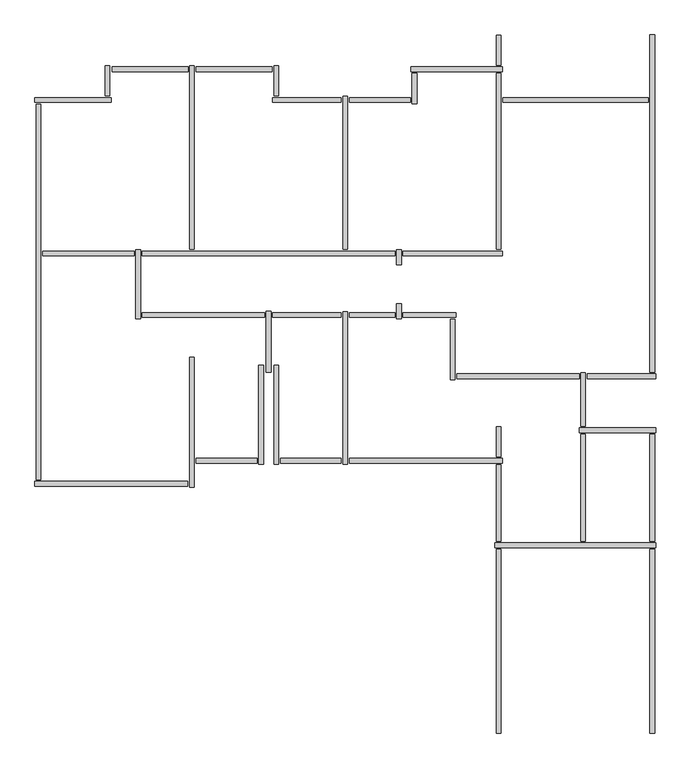
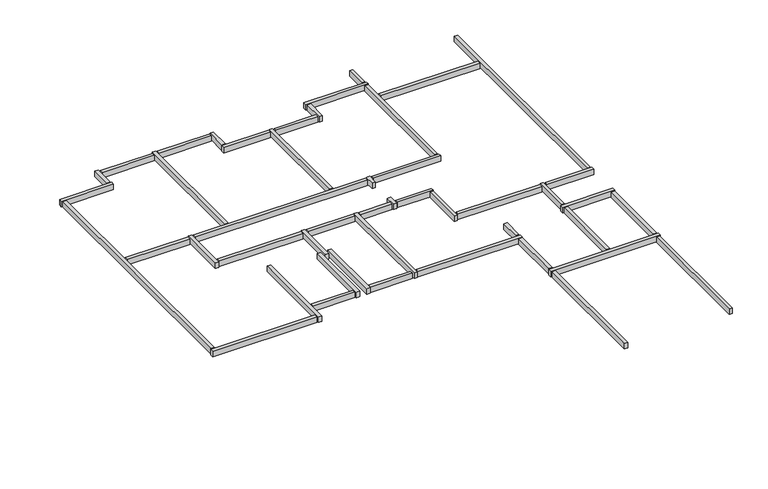
"""IFC4 building model written with IfcOpenShell, lengths in millimetres: beam geometry, Graute viga de respaldo23 : Graute viga de respaldo."""

from ifc_helpers import new_model, si_unit, frame, origin, place, context, project, spatial, polyline, outline, extrude, source, transform, mapped, element, save


def beam_4ae021a0(model_context):
    return source(origin(), model_context, "Body", "SweptSolid", [
        extrude(outline(polyline([(-70718.7587292, 62785.4278788), (-70624.7587292, 62785.4278788), (-70624.7587292, 59195.4278788), (-70718.7587292, 59195.4278788), (-70718.7587292, 62785.4278788)])), frame((0.0, 0.0, 17632.9999999), z_axis=(0.0, 0.0, 1.0), x_axis=(1.0, 0.0, 0.0)), (0.0, 0.0, 1.0), 167.0),
        extrude(outline(polyline([(-67718.7587292, 62785.4278788), (-67624.7587292, 62785.4278788), (-67624.7587292, 59195.4278788), (-67718.7587292, 59195.4278788), (-67718.7587292, 62785.4278788)])), frame((0.0, 0.0, 17632.9999999), z_axis=(0.0, 0.0, 1.0), x_axis=(1.0, 0.0, 0.0)), (0.0, 0.0, 1.0), 167.0),
        extrude(outline(polyline([(-75401.7587292, 64562.4278788), (-75401.7587292, 64468.4278788), (-76591.7587292, 64468.4278788), (-76591.7587292, 64562.4278788), (-75401.7587292, 64562.4278788)])), frame((0.0, 0.0, 17632.9999999), z_axis=(0.0, 0.0, 1.0), x_axis=(1.0, 0.0, 0.0)), (0.0, 0.0, 1.0), 167.0),
        extrude(outline(polyline([(-73751.7587292, 64562.4278788), (-73751.7587292, 64468.4278788), (-74941.7587292, 64468.4278788), (-74941.7587292, 64562.4278788), (-73751.7587292, 64562.4278788)])), frame((0.0, 0.0, 17632.9999999), z_axis=(0.0, 0.0, 1.0), x_axis=(1.0, 0.0, 0.0)), (0.0, 0.0, 1.0), 167.0),
        extrude(outline(polyline([(-77801.7587292, 68612.4278788), (-77801.7587292, 68518.4278788), (-79591.7587292, 68518.4278788), (-79591.7587292, 68612.4278788), (-77801.7587292, 68612.4278788)])), frame((0.0, 0.0, 17632.9999999), z_axis=(0.0, 0.0, 1.0), x_axis=(1.0, 0.0, 0.0)), (0.0, 0.0, 1.0), 167.0),
        extrude(outline(polyline([(-72401.7587292, 71612.4278788), (-72401.7587292, 71518.4278788), (-73591.7587292, 71518.4278788), (-73591.7587292, 71612.4278788), (-72401.7587292, 71612.4278788)])), frame((0.0, 0.0, 17632.9999999), z_axis=(0.0, 0.0, 1.0), x_axis=(1.0, 0.0, 0.0)), (0.0, 0.0, 1.0), 167.0),
        extrude(outline(polyline([(-72274.7587292, 71495.4278788), (-72368.7587292, 71495.4278788), (-72368.7587292, 72085.4278788), (-72274.7587292, 72085.4278788), (-72274.7587292, 71495.4278788)])), frame((0.0, 0.0, 17632.9999999), z_axis=(0.0, 0.0, 1.0), x_axis=(1.0, 0.0, 0.0)), (0.0, 0.0, 1.0), 167.0),
        extrude(outline(polyline([(-70601.7587292, 72212.4278788), (-70601.7587292, 72118.4278788), (-72391.7587292, 72118.4278788), (-72391.7587292, 72212.4278788), (-70601.7587292, 72212.4278788)])), frame((0.0, 0.0, 17632.9999999), z_axis=(0.0, 0.0, 1.0), x_axis=(1.0, 0.0, 0.0)), (0.0, 0.0, 1.0), 167.0),
        extrude(outline(polyline([(-72668.7587292, 68635.4278788), (-72574.7587292, 68635.4278788), (-72574.7587292, 68345.4278788), (-72668.7587292, 68345.4278788), (-72668.7587292, 68635.4278788)])), frame((0.0, 0.0, 17632.9999999), z_axis=(0.0, 0.0, 1.0), x_axis=(1.0, 0.0, 0.0)), (0.0, 0.0, 1.0), 167.0),
        extrude(outline(polyline([(-75251.7587292, 67412.4278788), (-75251.7587292, 67318.4278788), (-77641.7587292, 67318.4278788), (-77641.7587292, 67412.4278788), (-75251.7587292, 67412.4278788)])), frame((0.0, 0.0, 17632.9999999), z_axis=(0.0, 0.0, 1.0), x_axis=(1.0, 0.0, 0.0)), (0.0, 0.0, 1.0), 167.0),
        extrude(outline(polyline([(-73751.7587292, 67412.4278788), (-73751.7587292, 67318.4278788), (-75091.7587292, 67318.4278788), (-75091.7587292, 67412.4278788), (-73751.7587292, 67412.4278788)])), frame((0.0, 0.0, 17632.9999999), z_axis=(0.0, 0.0, 1.0), x_axis=(1.0, 0.0, 0.0)), (0.0, 0.0, 1.0), 167.0),
        extrude(outline(polyline([(-72701.7587292, 67412.4278788), (-72701.7587292, 67318.4278788), (-73591.7587292, 67318.4278788), (-73591.7587292, 67412.4278788), (-72701.7587292, 67412.4278788)])), frame((0.0, 0.0, 17632.9999999), z_axis=(0.0, 0.0, 1.0), x_axis=(1.0, 0.0, 0.0)), (0.0, 0.0, 1.0), 167.0),
        extrude(outline(polyline([(-72668.7587292, 67585.4278788), (-72574.7587292, 67585.4278788), (-72574.7587292, 67295.4278788), (-72668.7587292, 67295.4278788), (-72668.7587292, 67585.4278788)])), frame((0.0, 0.0, 17632.9999999), z_axis=(0.0, 0.0, 1.0), x_axis=(1.0, 0.0, 0.0)), (0.0, 0.0, 1.0), 167.0),
        extrude(outline(polyline([(-71511.7587292, 67412.4278788), (-71511.7587292, 67318.4278788), (-72541.7587292, 67318.4278788), (-72541.7587292, 67412.4278788), (-71511.7587292, 67412.4278788)])), frame((0.0, 0.0, 17632.9999999), z_axis=(0.0, 0.0, 1.0), x_axis=(1.0, 0.0, 0.0)), (0.0, 0.0, 1.0), 167.0),
        extrude(outline(polyline([(-71524.7587292, 66095.4278788), (-71618.7587292, 66095.4278788), (-71618.7587292, 67285.4278788), (-71524.7587292, 67285.4278788), (-71524.7587292, 66095.4278788)])), frame((0.0, 0.0, 17632.9999999), z_axis=(0.0, 0.0, 1.0), x_axis=(1.0, 0.0, 0.0)), (0.0, 0.0, 1.0), 167.0),
        extrude(outline(polyline([(-69091.7587292, 66212.4278788), (-69091.7587292, 66118.4278788), (-71491.7587292, 66118.4278788), (-71491.7587292, 66212.4278788), (-69091.7587292, 66212.4278788)])), frame((0.0, 0.0, 17632.9999999), z_axis=(0.0, 0.0, 1.0), x_axis=(1.0, 0.0, 0.0)), (0.0, 0.0, 1.0), 167.0),
        extrude(outline(polyline([(-73718.7587292, 67430.4278788), (-73624.7587292, 67430.4278788), (-73624.7587292, 64445.4278788), (-73718.7587292, 64445.4278788), (-73718.7587292, 67430.4278788)])), frame((0.0, 0.0, 17632.9999999), z_axis=(0.0, 0.0, 1.0), x_axis=(1.0, 0.0, 0.0)), (0.0, 0.0, 1.0), 167.0),
        extrude(outline(polyline([(-70601.7587292, 64562.4278788), (-70601.7587292, 64468.4278788), (-73591.7587292, 64468.4278788), (-73591.7587292, 64562.4278788), (-70601.7587292, 64562.4278788)])), frame((0.0, 0.0, 17632.9999999), z_axis=(0.0, 0.0, 1.0), x_axis=(1.0, 0.0, 0.0)), (0.0, 0.0, 1.0), 167.0),
        extrude(outline(polyline([(-70718.7587292, 65185.4278788), (-70624.7587292, 65185.4278788), (-70624.7587292, 64595.4278788), (-70718.7587292, 64595.4278788), (-70718.7587292, 65185.4278788)])), frame((0.0, 0.0, 17632.9999999), z_axis=(0.0, 0.0, 1.0), x_axis=(1.0, 0.0, 0.0)), (0.0, 0.0, 1.0), 167.0),
        extrude(outline(polyline([(-70624.7587292, 62945.4278788), (-70718.7587292, 62945.4278788), (-70718.7587292, 64435.4278788), (-70624.7587292, 64435.4278788), (-70624.7587292, 62945.4278788)])), frame((0.0, 0.0, 17632.9999999), z_axis=(0.0, 0.0, 1.0), x_axis=(1.0, 0.0, 0.0)), (0.0, 0.0, 1.0), 167.0),
        extrude(outline(polyline([(-67624.7587292, 62945.4278788), (-67718.7587292, 62945.4278788), (-67718.7587292, 65035.4278788), (-67624.7587292, 65035.4278788), (-67624.7587292, 62945.4278788)])), frame((0.0, 0.0, 17632.9999999), z_axis=(0.0, 0.0, 1.0), x_axis=(1.0, 0.0, 0.0)), (0.0, 0.0, 1.0), 167.0),
        extrude(outline(polyline([(-68974.7587292, 62945.4278788), (-69068.7587292, 62945.4278788), (-69068.7587292, 65035.4278788), (-68974.7587292, 65035.4278788), (-68974.7587292, 62945.4278788)])), frame((0.0, 0.0, 17632.9999999), z_axis=(0.0, 0.0, 1.0), x_axis=(1.0, 0.0, 0.0)), (0.0, 0.0, 1.0), 167.0),
        extrude(outline(polyline([(-69068.7587292, 66235.4278788), (-68974.7587292, 66235.4278788), (-68974.7587292, 65195.4278788), (-69068.7587292, 65195.4278788), (-69068.7587292, 66235.4278788)])), frame((0.0, 0.0, 17632.9999999), z_axis=(0.0, 0.0, 1.0), x_axis=(1.0, 0.0, 0.0)), (0.0, 0.0, 1.0), 167.0),
        extrude(outline(polyline([(-67751.7587292, 71612.4278788), (-67751.7587292, 71518.4278788), (-70591.7587292, 71518.4278788), (-70591.7587292, 71612.4278788), (-67751.7587292, 71612.4278788)])), frame((0.0, 0.0, 17632.9999999), z_axis=(0.0, 0.0, 1.0), x_axis=(1.0, 0.0, 0.0)), (0.0, 0.0, 1.0), 167.0),
        extrude(outline(polyline([(-70624.7587292, 68645.4278788), (-70718.7587292, 68645.4278788), (-70718.7587292, 72085.4278788), (-70624.7587292, 72085.4278788), (-70624.7587292, 68645.4278788)])), frame((0.0, 0.0, 17632.9999999), z_axis=(0.0, 0.0, 1.0), x_axis=(1.0, 0.0, 0.0)), (0.0, 0.0, 1.0), 167.0),
        extrude(outline(polyline([(-70601.7587292, 68612.4278788), (-70601.7587292, 68518.4278788), (-72541.7587292, 68518.4278788), (-72541.7587292, 68612.4278788), (-70601.7587292, 68612.4278788)])), frame((0.0, 0.0, 17632.9999999), z_axis=(0.0, 0.0, 1.0), x_axis=(1.0, 0.0, 0.0)), (0.0, 0.0, 1.0), 167.0),
        extrude(outline(polyline([(-72701.7587292, 68612.4278788), (-72701.7587292, 68518.4278788), (-77641.7587292, 68518.4278788), (-77641.7587292, 68612.4278788), (-72701.7587292, 68612.4278788)])), frame((0.0, 0.0, 17632.9999999), z_axis=(0.0, 0.0, 1.0), x_axis=(1.0, 0.0, 0.0)), (0.0, 0.0, 1.0), 167.0),
        extrude(outline(polyline([(-73718.7587292, 71635.4278788), (-73624.7587292, 71635.4278788), (-73624.7587292, 68645.4278788), (-73718.7587292, 68645.4278788), (-73718.7587292, 71635.4278788)])), frame((0.0, 0.0, 17632.9999999), z_axis=(0.0, 0.0, 1.0), x_axis=(1.0, 0.0, 0.0)), (0.0, 0.0, 1.0), 167.0),
        extrude(outline(polyline([(-75091.7587292, 71518.4278788), (-75091.7587292, 71612.4278788), (-73751.7587292, 71612.4278788), (-73751.7587292, 71518.4278788), (-75091.7587292, 71518.4278788)])), frame((0.0, 0.0, 17632.9999999), z_axis=(0.0, 0.0, 1.0), x_axis=(1.0, 0.0, 0.0)), (0.0, 0.0, 1.0), 167.0),
        extrude(outline(polyline([(-75068.7587292, 72235.4278788), (-74974.7587292, 72235.4278788), (-74974.7587292, 71645.4278788), (-75068.7587292, 71645.4278788), (-75068.7587292, 72235.4278788)])), frame((0.0, 0.0, 17632.9999999), z_axis=(0.0, 0.0, 1.0), x_axis=(1.0, 0.0, 0.0)), (0.0, 0.0, 1.0), 167.0),
        extrude(outline(polyline([(-75101.7587292, 72212.4278788), (-75101.7587292, 72118.4278788), (-76591.7587292, 72118.4278788), (-76591.7587292, 72212.4278788), (-75101.7587292, 72212.4278788)])), frame((0.0, 0.0, 17632.9999999), z_axis=(0.0, 0.0, 1.0), x_axis=(1.0, 0.0, 0.0)), (0.0, 0.0, 1.0), 167.0),
        extrude(outline(polyline([(-78230.736554, 72117.4278788), (-78230.736554, 72212.4278788), (-76741.7587292, 72212.4278788), (-76741.7587292, 72117.4278788), (-78230.736554, 72117.4278788)])), frame((0.0, 0.0, 17617.1856208), z_axis=(0.0, 0.0, 1.0), x_axis=(1.0, 0.0, 0.0)), (0.0, 0.0, 1.0), 165.0),
        extrude(outline(polyline([(-79624.7587292, 64145.4278788), (-79718.7587292, 64145.4278788), (-79718.7587292, 71485.4278788), (-79624.7587292, 71485.4278788), (-79624.7587292, 64145.4278788)])), frame((0.0, 0.0, 17632.9999999), z_axis=(0.0, 0.0, 1.0), x_axis=(1.0, 0.0, 0.0)), (0.0, 0.0, 1.0), 167.0),
        extrude(outline(polyline([(-77674.7587292, 67295.4278788), (-77768.7587292, 67295.4278788), (-77768.7587292, 68640.7810915), (-77674.7587292, 68640.7810915), (-77674.7587292, 67295.4278788)])), frame((0.0, 0.0, 17632.9999999), z_axis=(0.0, 0.0, 1.0), x_axis=(1.0, 0.0, 0.0)), (0.0, 0.0, 1.0), 167.0),
        extrude(outline(polyline([(-75124.7587292, 66245.4278788), (-75218.7587292, 66245.4278788), (-75218.7587292, 67435.4278788), (-75124.7587292, 67435.4278788), (-75124.7587292, 66245.4278788)])), frame((0.0, 0.0, 17632.9999999), z_axis=(0.0, 0.0, 1.0), x_axis=(1.0, 0.0, 0.0)), (0.0, 0.0, 1.0), 167.0),
        extrude(outline(polyline([(-75274.7587292, 64445.4278788), (-75368.7587292, 64445.4278788), (-75368.7587292, 66385.4278788), (-75274.7587292, 66385.4278788), (-75274.7587292, 64445.4278788)])), frame((0.0, 0.0, 17632.9999999), z_axis=(0.0, 0.0, 1.0), x_axis=(1.0, 0.0, 0.0)), (0.0, 0.0, 1.0), 167.0),
        extrude(outline(polyline([(-74974.7587292, 64445.4278788), (-75068.7587292, 64445.4278788), (-75068.7587292, 66385.4278788), (-74974.7587292, 66385.4278788), (-74974.7587292, 64445.4278788)])), frame((0.0, 0.0, 17632.9999999), z_axis=(0.0, 0.0, 1.0), x_axis=(1.0, 0.0, 0.0)), (0.0, 0.0, 1.0), 167.0),
        extrude(outline(polyline([(-76624.7587292, 63995.4278788), (-76718.7587292, 63995.4278788), (-76718.7587292, 66535.4278788), (-76624.7587292, 66535.4278788), (-76624.7587292, 63995.4278788)])), frame((0.0, 0.0, 17632.9999999), z_axis=(0.0, 0.0, 1.0), x_axis=(1.0, 0.0, 0.0)), (0.0, 0.0, 1.0), 167.0),
        extrude(outline(polyline([(-79741.7587292, 64018.4278788), (-79741.7587292, 64112.4278788), (-76751.7587292, 64112.4278788), (-76751.7587292, 64018.4278788), (-79741.7587292, 64018.4278788)])), frame((0.0, 0.0, 17632.9999999), z_axis=(0.0, 0.0, 1.0), x_axis=(1.0, 0.0, 0.0)), (0.0, 0.0, 1.0), 167.0),
        extrude(outline(polyline([(-78368.7587292, 72235.4278788), (-78274.7587292, 72235.4278788), (-78274.7587292, 71645.4278788), (-78368.7587292, 71645.4278788), (-78368.7587292, 72235.4278788)])), frame((0.0, 0.0, 17632.9999999), z_axis=(0.0, 0.0, 1.0), x_axis=(1.0, 0.0, 0.0)), (0.0, 0.0, 1.0), 167.0),
        extrude(outline(polyline([(-78251.7587292, 71612.4278788), (-78251.7587292, 71518.4278788), (-79741.7587292, 71518.4278788), (-79741.7587292, 71612.4278788), (-78251.7587292, 71612.4278788)])), frame((0.0, 0.0, 17632.9999999), z_axis=(0.0, 0.0, 1.0), x_axis=(1.0, 0.0, 0.0)), (0.0, 0.0, 1.0), 167.0),
        extrude(outline(polyline([(-76718.7587292, 72235.4278788), (-76624.7587292, 72235.4278788), (-76624.7587292, 68645.4278788), (-76718.7587292, 68645.4278788), (-76718.7587292, 72235.4278788)])), frame((0.0, 0.0, 17632.9999999), z_axis=(0.0, 0.0, 1.0), x_axis=(1.0, 0.0, 0.0)), (0.0, 0.0, 1.0), 167.0),
        extrude(outline(polyline([(-70718.7587292, 72835.4278788), (-70624.7587292, 72835.4278788), (-70624.7587292, 72245.4278788), (-70718.7587292, 72245.4278788), (-70718.7587292, 72835.4278788)])), frame((0.0, 0.0, 17632.9999999), z_axis=(0.0, 0.0, 1.0), x_axis=(1.0, 0.0, 0.0)), (0.0, 0.0, 1.0), 167.0),
        extrude(outline(polyline([(-67601.7587292, 65162.4278788), (-67601.7587292, 65068.4278788), (-69091.7587292, 65068.4278788), (-69091.7587292, 65162.4278788), (-67601.7587292, 65162.4278788)])), frame((0.0, 0.0, 17632.9999999), z_axis=(0.0, 0.0, 1.0), x_axis=(1.0, 0.0, 0.0)), (0.0, 0.0, 1.0), 167.0),
        extrude(outline(polyline([(-67601.7587292, 62912.4278788), (-67601.7587292, 62818.4278788), (-70741.7587292, 62818.4278788), (-70741.7587292, 62912.4278788), (-67601.7587292, 62912.4278788)])), frame((0.0, 0.0, 17632.9999999), z_axis=(0.0, 0.0, 1.0), x_axis=(1.0, 0.0, 0.0)), (0.0, 0.0, 1.0), 167.0),
        extrude(outline(polyline([(-67601.7587292, 66212.4278788), (-67601.7587292, 66118.4278788), (-68941.7587292, 66118.4278788), (-68941.7587292, 66212.4278788), (-67601.7587292, 66212.4278788)])), frame((0.0, 0.0, 17632.9999999), z_axis=(0.0, 0.0, 1.0), x_axis=(1.0, 0.0, 0.0)), (0.0, 0.0, 1.0), 167.0),
        extrude(outline(polyline([(-67718.7587292, 72837.9577736), (-67624.7587292, 72837.9577736), (-67624.7587292, 66245.4278788), (-67718.7587292, 66245.4278788), (-67718.7587292, 72837.9577736)])), frame((0.0, 0.0, 17632.9999999), z_axis=(0.0, 0.0, 1.0), x_axis=(1.0, 0.0, 0.0)), (0.0, 0.0, 1.0), 167.0),
    ])


if __name__ == "__main__":
    model = new_model("IFC4")
    model_context = context("Model", 3, world=origin())
    ifc_project = project(units=[si_unit("LENGTHUNIT", "METRE", prefix="MILLI")], contexts=[model_context])
    site = spatial("IfcSite", under=ifc_project)
    building = spatial("IfcBuilding", under=site)
    placement = place(None, origin())
    beam_shape = beam_4ae021a0(model_context)
    element("IfcBeam", 1, ObjectType="Graute viga de respaldo23 : Graute viga de respaldo", at=placement, inside=building, context=model_context, shape_type="MappedRepresentation", body=[
        mapped(beam_shape, transform((0.0, 0.0, 0.0), x_axis=(1.0, 0.0, 0.0), y_axis=(0.0, 1.0, 0.0), z_axis=(0.0, 0.0, 1.0))),
    ])
    save(model, "model.ifc")

# Revit data of these elements
# Element 1 (IfcBeam, "Graute viga de respaldo23 : Graute viga de respaldo")
#   Materials on its faces: "Concreto, Faixa de areia/cimento"
# Materials
#   "Concreto, Faixa de areia/cimento": class "Concreto", colour RGB 127 127 127, transparency 0, Description = "Revestimento de laje de concreto", Cost = 0
